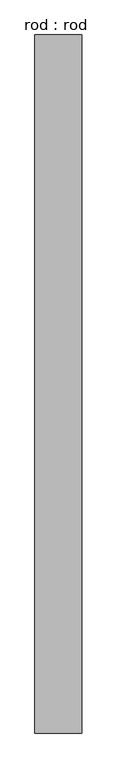
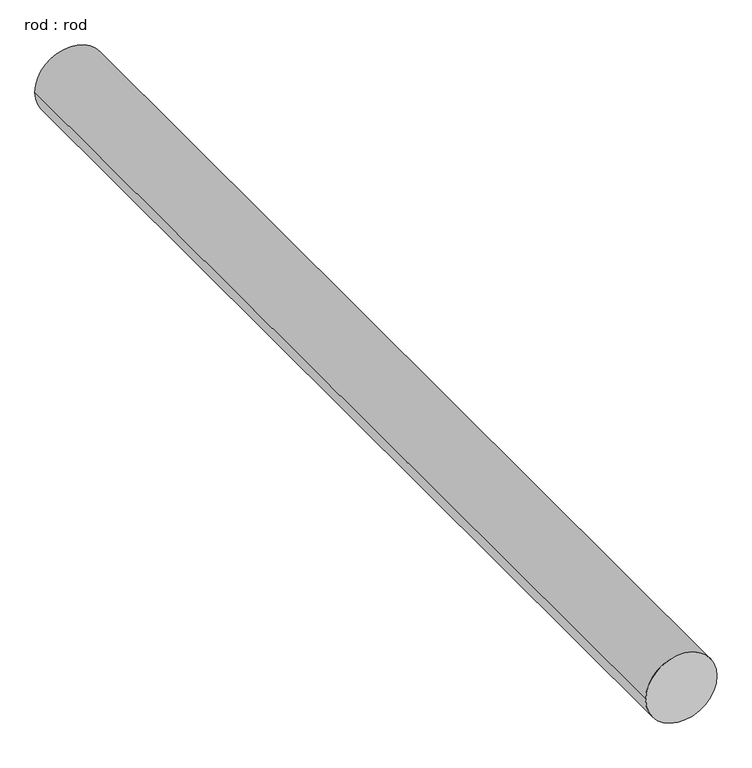
"""IFC4 building model written with IfcOpenShell, lengths in millimetres: proxy geometry, rod : rod."""

from ifc_helpers import new_model, si_unit, point, frame, frame_2d, origin, place, context, project, spatial, circle_curve, trimmed, segment, composite_curve, outline, extrude, source, transform, mapped, element, save


def rod_rod_f0e88d89(model_context):
    return source(origin(), model_context, "Body", "SweptSolid", [
        extrude(outline(composite_curve([segment(trimmed(circle_curve(frame_2d((0.0108462, 0.0)), 200.0), [point((0.0108462, 200.0))], [point((0.0108462, -200.0))], False, "CARTESIAN"), True, "CONTINUOUS"), segment(trimmed(circle_curve(frame_2d((0.0108462, 0.0)), 200.0), [point((0.0108462, -200.0))], [point((0.0108462, 200.0))], False, "CARTESIAN"), True, "CONTINUOUS")], self_intersect=False)), frame((0.0, 1119.3565636, 0.0), z_axis=(0.0, 1.0, 0.0), x_axis=(0.0, 0.0, 1.0)), (0.0, 0.0, 1.0), 5946.7441035),
    ])


if __name__ == "__main__":
    model = new_model("IFC4")
    model_context = context("Model", 3, world=origin())
    ifc_project = project(units=[si_unit("LENGTHUNIT", "METRE", prefix="MILLI")], contexts=[model_context])
    site = spatial("IfcSite", under=ifc_project)
    building = spatial("IfcBuilding", under=site)
    placement = place(None, origin())
    rod_rod_shape = rod_rod_f0e88d89(model_context)
    element("IfcBuildingElementProxy", 1, Name="rod : rod", ObjectType="rod : rod", at=placement, inside=building, context=model_context, shape_type="MappedRepresentation", body=[
        mapped(rod_rod_shape, transform((0.0, 0.0, 0.0), x_axis=(1.0, 0.0, 0.0), y_axis=(0.0, 1.0, 0.0), z_axis=(0.0, 0.0, 1.0))),
    ])
    save(model, "model.ifc")

# Revit data of these elements
# Type "rod : rod"
#   Default Elevation = 0
